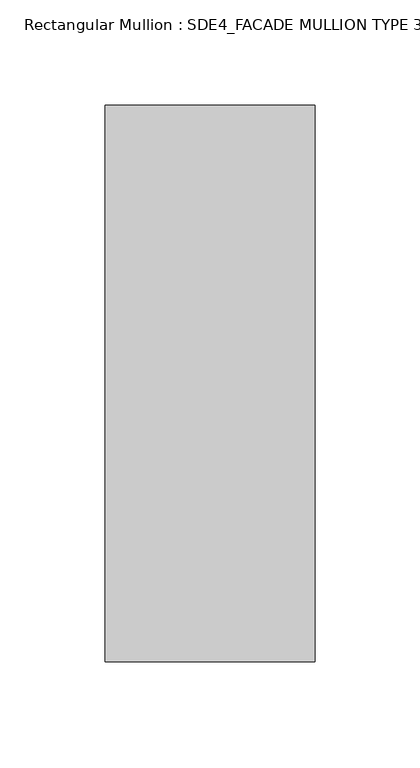
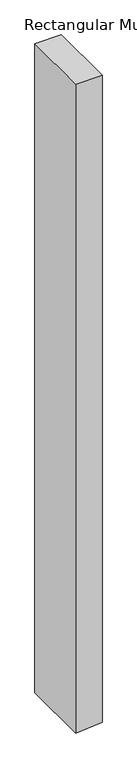
"""IFC4 building model written with IfcOpenShell, lengths in millimetres: member geometry, Rectangular Mullion : SDE4_FACADE MULLION TYPE 3."""

from ifc_helpers import new_model, si_unit, frame, origin, place, context, project, spatial, polyline, outline, extrude, source, transform, mapped, element, save


def rectangular_mullion_sde4_facade_mullion_type_3_20fab93c(model_context):
    return source(origin(), model_context, "Body", "SweptSolid", [
        extrude(outline(polyline([(0.0, 50.0), (0.0, -50.0), (-2586.163656, -50.0), (-2582.5660587, -3.056508), (-2578.4999796, 50.0), (0.0, 50.0)])), frame((0.0, -132.5, 0.0), z_axis=(0.0, 1.0, 0.0), x_axis=(0.0, 0.0, 1.0)), (0.0, 0.0, 1.0), 265.0),
    ])


if __name__ == "__main__":
    model = new_model("IFC4")
    model_context = context("Model", 3, world=origin())
    ifc_project = project(units=[si_unit("LENGTHUNIT", "METRE", prefix="MILLI")], contexts=[model_context])
    site = spatial("IfcSite", under=ifc_project)
    building = spatial("IfcBuilding", under=site)
    placement = place(None, origin())
    rectangular_mullion_sde4_facade_mullion_type_3_shape = rectangular_mullion_sde4_facade_mullion_type_3_20fab93c(model_context)
    element("IfcMember", 1, ObjectType="Rectangular Mullion : SDE4_FACADE MULLION TYPE 3", at=placement, inside=building, context=model_context, shape_type="MappedRepresentation", body=[
        mapped(rectangular_mullion_sde4_facade_mullion_type_3_shape, transform((0.0, 0.0, 0.0), x_axis=(1.0, 0.0, 0.0), y_axis=(0.0, 1.0, 0.0), z_axis=(0.0, 0.0, 1.0))),
    ])
    save(model, "model.ifc")

# Revit data of these elements
# Type "Rectangular Mullion : SDE4_FACADE MULLION TYPE 3"
#   built-in parameter 1007322 = 0.869423 (stored number, unit not read)
#   built-in parameter 1007321 = 0.164042 (stored number, unit not read)
#   built-in parameter 1007320 = 0.164042 (stored number, unit not read)
